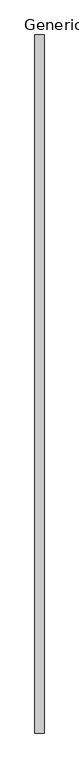
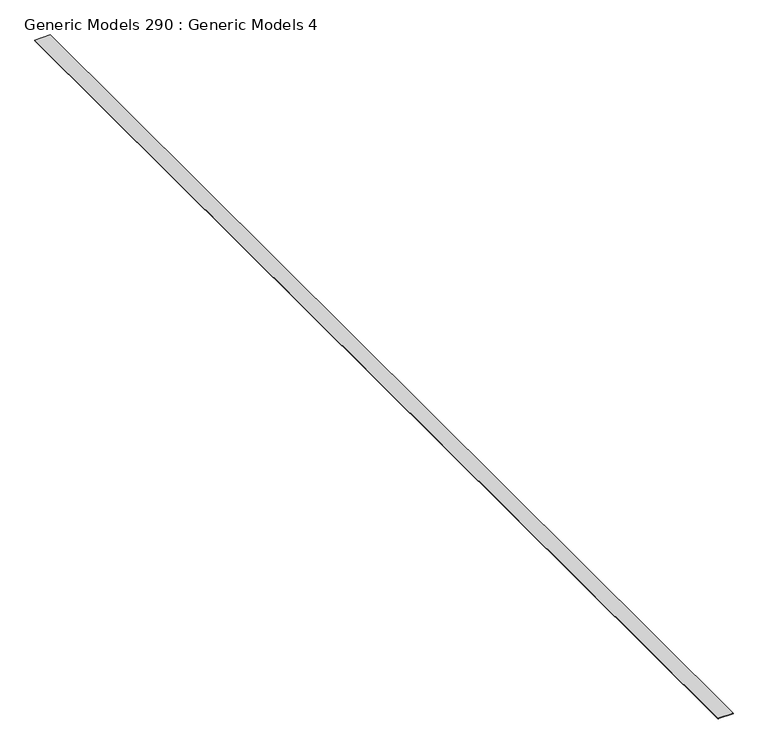
"""IFC4 building model written with IfcOpenShell, lengths in millimetres: proxy geometry, Generic Models 290 : Generic Models 4."""

from ifc_helpers import new_model, si_unit, frame, origin, place, context, project, spatial, polyline, outline, extrude, source, transform, mapped, element, save


def generic_models_290_generic_models_4_8ceec6c9(model_context):
    return source(origin(), model_context, "Body", "SweptSolid", [
        extrude(outline(polyline([(87307.251867, 24984.1772257), (87410.4113509, 24984.1772257), (87410.4113509, 17097.4772257), (87307.251867, 17097.4772257), (87307.251867, 24984.1772257)])), frame((0.0, 0.0, 123328.7508022), z_axis=(0.0, 0.0, 1.0), x_axis=(1.0, 0.0, 0.0)), (0.0, 0.0, 1.0), 1.3753749),
        extrude(outline(polyline([(87307.251867, 24984.1772257), (87410.4113509, 24984.1772257), (87410.4113509, 17097.4772257), (87307.251867, 17097.4772257), (87307.251867, 24984.1772257)])), frame((0.0, 0.0, 123325.357144), z_axis=(0.0, 0.0, 1.0), x_axis=(1.0, 0.0, 0.0)), (0.0, 0.0, 1.0), 1.3753749),
    ])


if __name__ == "__main__":
    model = new_model("IFC4")
    model_context = context("Model", 3, world=origin())
    ifc_project = project(units=[si_unit("LENGTHUNIT", "METRE", prefix="MILLI")], contexts=[model_context])
    site = spatial("IfcSite", under=ifc_project)
    building = spatial("IfcBuilding", under=site)
    placement = place(None, origin())
    generic_models_290_generic_models_4_shape = generic_models_290_generic_models_4_8ceec6c9(model_context)
    element("IfcBuildingElementProxy", 1, Name="Generic Models 290 : Generic Models 4", ObjectType="Generic Models 290 : Generic Models 4", at=placement, inside=building, context=model_context, shape_type="MappedRepresentation", body=[
        mapped(generic_models_290_generic_models_4_shape, transform((0.0, 0.0, 0.0), x_axis=(1.0, 0.0, 0.0), y_axis=(0.0, 1.0, 0.0), z_axis=(0.0, 0.0, 1.0))),
    ])
    save(model, "model.ifc")

# Revit data of these elements
# Element 1 (IfcBuildingElementProxy, "Generic Models 290 : Generic Models 4")
#   Materials on its faces: "_BED OF SEALANT (ABOVE/BELOW FLASHING)"
# Materials
#   "_BED OF SEALANT (ABOVE/BELOW FLASHING)": class "Generic", colour RGB 253 192 103, transparency 0, Cost = 0
